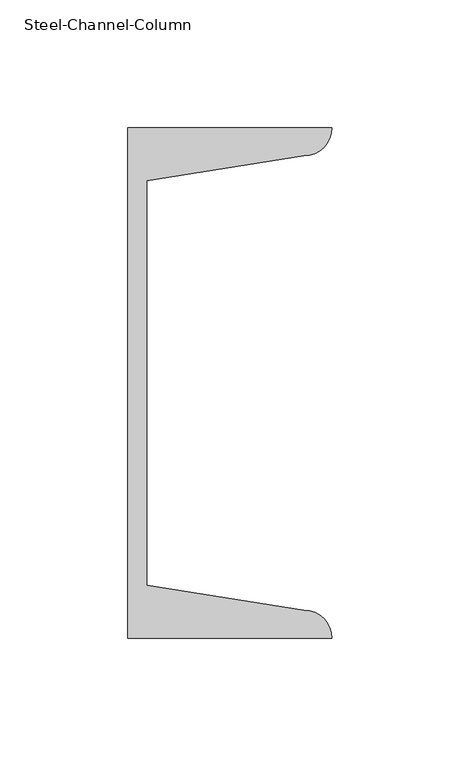
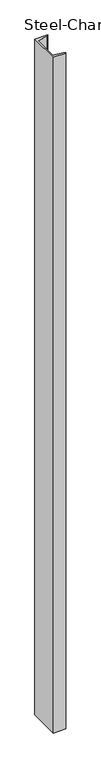
"""IFC4 building model written with IfcOpenShell, lengths in millimetres: column geometry, Steel-Channel-Column : CL126_C-200×80x7.5x11."""

from ifc_helpers import new_model, si_unit, point, frame_2d, origin, origin_with_axes, place, context, project, spatial, polyline, circle_curve, trimmed, segment, composite_curve, outline, extrude, source, transform, mapped, element, save


def steel_channel_column_e5f447b6(model_context):
    return source(origin(), model_context, "Body", "SweptSolid", [
        extrude(outline(composite_curve([segment(polyline([(-22.1, -100.0), (-22.1, 100.0), (57.9, 100.0)]), True, "CONTINUOUS"), segment(trimmed(circle_curve(frame_2d((46.9, 100.0)), 11.0), [point((57.9, 100.0))], [point((46.9, 89.0))], False, "CARTESIAN"), True, "CONTINUOUS"), segment(polyline([(46.9, 89.0), (-14.6, 79.2593569), (-14.6, -79.2593569), (46.9, -89.0)]), True, "CONTINUOUS"), segment(trimmed(circle_curve(frame_2d((46.9, -100.0)), 11.0), [point((46.9, -89.0))], [point((57.9, -100.0))], False, "CARTESIAN"), True, "CONTINUOUS"), segment(polyline([(57.9, -100.0), (-22.1, -100.0)]), True, "CONTINUOUS")], self_intersect=False)), origin_with_axes(), (0.0, 0.0, 1.0), 4500.0),
    ])


if __name__ == "__main__":
    model = new_model("IFC4")
    model_context = context("Model", 3, world=origin())
    ifc_project = project(units=[si_unit("LENGTHUNIT", "METRE", prefix="MILLI")], contexts=[model_context])
    site = spatial("IfcSite", under=ifc_project)
    building = spatial("IfcBuilding", under=site)
    placement = place(None, origin())
    steel_channel_column_shape = steel_channel_column_e5f447b6(model_context)
    element("IfcColumn", 1, ObjectType="Steel-Channel-Column : CL126_C-200×80x7.5x11", at=placement, inside=building, context=model_context, shape_type="MappedRepresentation", body=[
        mapped(steel_channel_column_shape, transform((0.0, 0.0, 0.0), x_axis=(1.0, 0.0, 0.0), y_axis=(0.0, 1.0, 0.0), z_axis=(0.0, 0.0, 1.0))),
    ])
    save(model, "model.ifc")

# Revit data of these elements
# Type "Steel-Channel-Column : CL126_C-200×80x7.5x11"
#   Assembly Code = "B10"
#   x = 22.1 mm
#   Section Area = 31.33 cm²
#   Mass per Unit Length = 24.60 kg/m
#   bf = 80 mm
#   d = 200 mm
#   tf = 11 mm
#   tw = 7.5 mm
#   hec_material4 [instance default] = none
#   hec_material3 [instance default] = none
#   hec_material2 [instance default] = none
#   hec_material1 [instance default] = none
#   Structural Material [instance default] = Steel, 45-345
# Element 1 (IfcColumn, "Steel-Channel-Column : CL126_C-200×80x7.5x11")
#   Materials on its faces: "Steel, 45-345"
# Materials
#   "Steel, 45-345": class "Metal", colour RGB 189 187 185, transparency 0, Description = "Steel 345 MPa", Cost = 0
